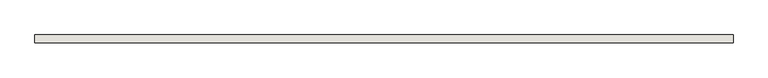
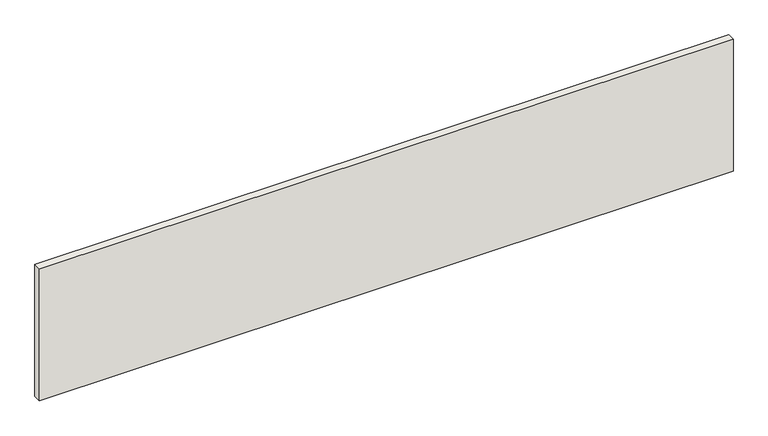
"""IFC4 building model written with IfcOpenShell, lengths in millimetres: wall geometry, Holzwand."""

from ifc_helpers import new_model, si_unit, origin, origin_with_axes, place, context, project, spatial, polyline, outline, extrude, source, transform, mapped, element, save


def wall_1d78180e(model_context):
    return source(origin(), model_context, "Body", "SweptSolid", [
        extrude(outline(polyline([(0.0, 50.0), (4469.8398546, 50.0), (4469.8398546, 0.0), (0.0, 0.0), (0.0, 50.0)])), origin_with_axes(), (0.0, 0.0, 1.0), 900.0),
    ])


if __name__ == "__main__":
    model = new_model("IFC4")
    model_context = context("Model", 3, world=origin())
    ifc_project = project(units=[si_unit("LENGTHUNIT", "METRE", prefix="MILLI")], contexts=[model_context])
    site = spatial("IfcSite", under=ifc_project)
    building = spatial("IfcBuilding", under=site)
    placement = place(None, origin())
    wall_shape = wall_1d78180e(model_context)
    element("IfcWall", 1, ObjectType="Holzwand", at=placement, inside=building, context=model_context, shape_type="MappedRepresentation", body=[
        mapped(wall_shape, transform((0.0, 0.0, 0.0), x_axis=(1.0, 0.0, 0.0), y_axis=(0.0, 1.0, 0.0), z_axis=(0.0, 0.0, 1.0))),
    ])
    save(model, "model.ifc")

# Revit data of these elements
# Element 1 (IfcWall, "Holzwand")
#   Materials on its faces: "holzschalung"
# Materials
#   "holzschalung": class "Unassigned", colour RGB 128 128 128, transparency 0
